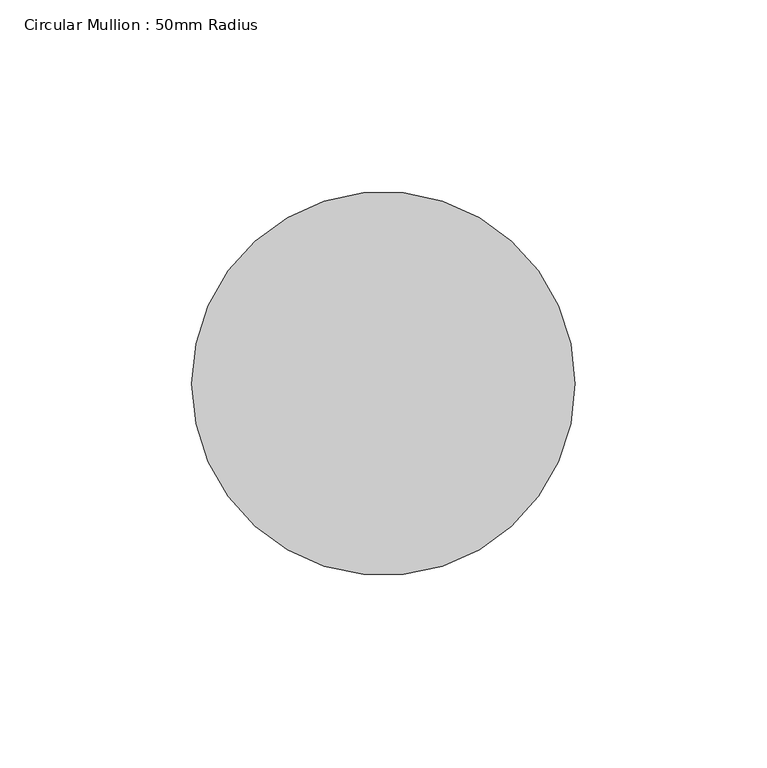
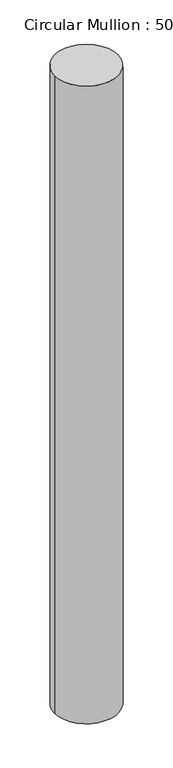
"""IFC4 building model written with IfcOpenShell, lengths in millimetres: member geometry, Circular Mullion : 50mm Radius."""

from ifc_helpers import new_model, si_unit, point, frame, origin, origin_2d, place, context, project, spatial, circle_curve, trimmed, segment, composite_curve, outline, extrude, source, transform, mapped, element, save


def circular_mullion_50mm_radius_68719307(model_context):
    return source(origin(), model_context, "Body", "SweptSolid", [
        extrude(outline(composite_curve([segment(trimmed(circle_curve(origin_2d(), 50.0), [point((50.0, 0.0))], [point((-50.0, 0.0))], False, "CARTESIAN"), True, "CONTINUOUS"), segment(trimmed(circle_curve(origin_2d(), 50.0), [point((-50.0, 0.0))], [point((50.0, 0.0))], False, "CARTESIAN"), True, "CONTINUOUS")], self_intersect=False)), frame((0.0, 0.0, -1064.1344929), z_axis=(0.0, 0.0, 1.0), x_axis=(1.0, 0.0, 0.0)), (0.0, 0.0, 1.0), 1064.1344929),
    ])


if __name__ == "__main__":
    model = new_model("IFC4")
    model_context = context("Model", 3, world=origin())
    ifc_project = project(units=[si_unit("LENGTHUNIT", "METRE", prefix="MILLI")], contexts=[model_context])
    site = spatial("IfcSite", under=ifc_project)
    building = spatial("IfcBuilding", under=site)
    placement = place(None, origin())
    circular_mullion_50mm_radius_shape = circular_mullion_50mm_radius_68719307(model_context)
    element("IfcMember", 1, ObjectType="Circular Mullion : 50mm Radius", at=placement, inside=building, context=model_context, shape_type="MappedRepresentation", body=[
        mapped(circular_mullion_50mm_radius_shape, transform((0.0, 0.0, 0.0), x_axis=(1.0, 0.0, 0.0), y_axis=(0.0, 1.0, 0.0), z_axis=(0.0, 0.0, 1.0))),
    ])
    save(model, "model.ifc")

# Revit data of these elements
# Type "Circular Mullion : 50mm Radius"
#   built-in parameter 1007350 = 0.164042 (stored number, unit not read)
# Element 1 (IfcMember, "Circular Mullion : 50mm Radius")
#   Materials on its faces: "Aluminium"
# Materials
#   "Aluminium": class "Metal", colour RGB 247 247 247, transparency 0, Description = "Aluminium 6061", Cost = 0
